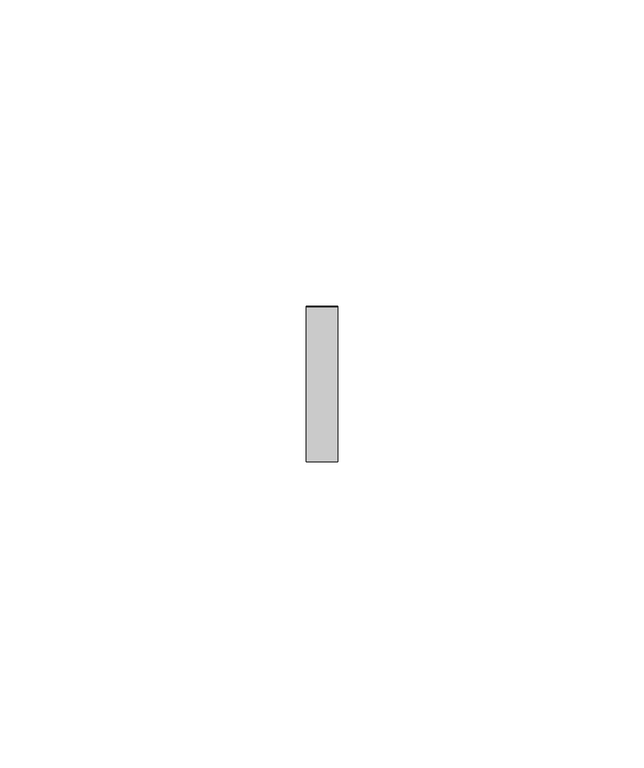
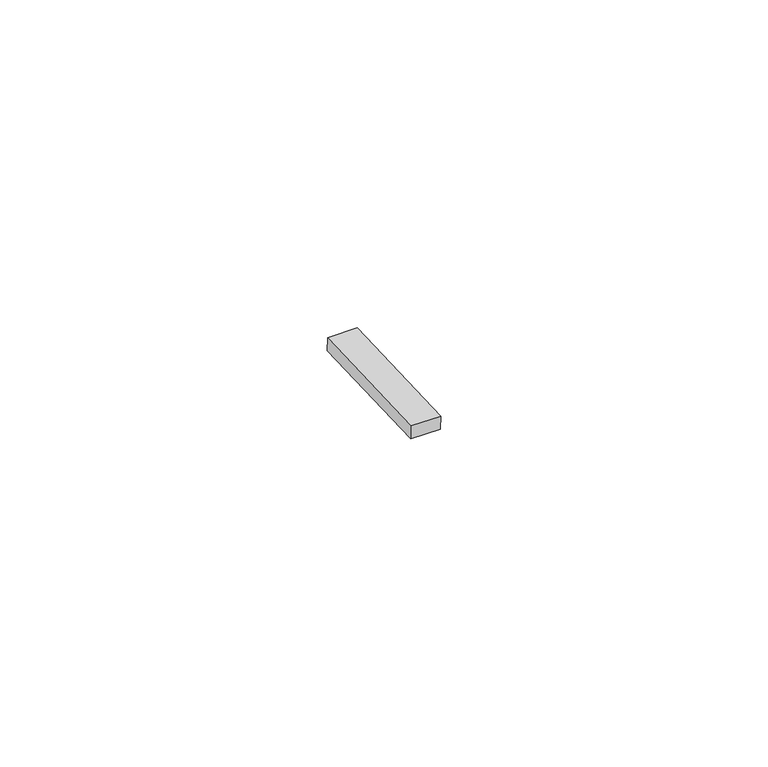
"""IFC4 building model written with IfcOpenShell, lengths in millimetres: proxy geometry, Inner panel:Inner panel:1:Inner panel:1 : Inner panel:Inner panel:300324:2:Inner panel:1:Inner panel:1 : Inner panel:Inner panel:300324:2 : Inner panel:Inner panel:1:Inner panel:1 : Inner panel:Inner panel:300324:300043:137 : Inner panel:Inner panel:1:Inner panel:1 : Inner panel:Inner panel:300324:2:Inner panel:1:Inner panel:1 : Inner panel:Inner panel:300324:2 : Inner panel:Inner panel:1:Inner panel:1 : Inner panel:Inner panel:300324:300043:308120."""

import ifcopenshell
import ifcopenshell.guid

model = None  # the IFC model being written
_history = None  # IfcOwnerHistory: only IFC2X3 demands one
_inside = {}  # id of a spatial element -> (the spatial element, [elements in it])
_under = {}  # id of a project, library or spatial element -> (it, [spatial elements below it])
_declared = {}  # id of a project -> (the project, [libraries it declares])
_typed = {}  # id of a type object -> (the type object, [elements of that type])
_made_of = {}  # id of a material, layer set ... -> (it, [elements and type objects made of it])


def new_model(schema):
    """Start an empty IFC model of exactly this schema.

    Asked for "IFC4X3", IfcOpenShell would pick the latest addendum, in which some entities
    have other attributes; the version numbers below select the first issue.
    IFC2X3 requires an IfcOwnerHistory on every rooted entity: one is made here for all.
    """
    global model, _history
    if schema == "IFC4X3":
        model = ifcopenshell.file(schema_version=(4, 3, 0, 0))
    else:
        model = ifcopenshell.file(schema=schema)
    _inside.clear()
    _under.clear()
    _declared.clear()
    _typed.clear()
    _made_of.clear()
    _history = None
    if model.schema == "IFC2X3":
        org = make("IfcOrganization", Name="unknown")
        user = make(
            "IfcPersonAndOrganization",
            ThePerson=make("IfcPerson", FamilyName="unknown"),
            TheOrganization=org,
        )
        app = make(
            "IfcApplication",
            ApplicationDeveloper=org,
            Version="unknown",
            ApplicationFullName="unknown",
            ApplicationIdentifier="unknown",
        )
        _history = make(
            "IfcOwnerHistory",
            OwningUser=user,
            OwningApplication=app,
            ChangeAction="ADDED",
            CreationDate=0,
        )
    return model


def make(cls, **values):
    """One entity of the class cls with the attributes given. An attribute that is None is left unset."""
    return model.create_entity(
        cls, **{name: value for name, value in values.items() if value is not None}
    )


def rooted(cls, **values):
    """An entity with a GlobalId (a new one), such as an element, a storey or a relation."""
    return make(cls, GlobalId=ifcopenshell.guid.new(), OwnerHistory=_history, **values)


def si_unit(unit_type, name, prefix=None):
    """IfcSIUnit, for example si_unit("LENGTHUNIT", "METRE", prefix="MILLI")."""
    return make("IfcSIUnit", UnitType=unit_type, Prefix=prefix, Name=name)


def assignment(units):
    """IfcUnitAssignment: the units of a project."""
    return None if units is None else make("IfcUnitAssignment", Units=units)


def point(xyz):
    """IfcCartesianPoint."""
    return None if xyz is None else make("IfcCartesianPoint", Coordinates=xyz)


def direction(xyz):
    """IfcDirection."""
    return None if xyz is None else make("IfcDirection", DirectionRatios=xyz)


def frame(location, z_axis=None, x_axis=None):
    """IfcAxis2Placement3D, a coordinate frame: its origin and axes. An axis left out is left unset."""
    return make(
        "IfcAxis2Placement3D",
        Location=point(location),
        Axis=direction(z_axis),
        RefDirection=direction(x_axis),
    )


def origin():
    """The frame at (0, 0, 0) with its axes left unset."""
    return frame((0.0, 0.0, 0.0))


def place(relative_to, where):
    """IfcLocalPlacement: puts the frame where relative to a parent placement (None: the world)."""
    return make(
        "IfcLocalPlacement", PlacementRelTo=relative_to, RelativePlacement=where
    )


def context(
    kind, dimensions, precision=None, world=None, true_north=None, identifier=None
):
    """IfcGeometricRepresentationContext, for example the 3D "Model" context."""
    return make(
        "IfcGeometricRepresentationContext",
        ContextIdentifier=identifier,
        ContextType=kind,
        CoordinateSpaceDimension=dimensions,
        Precision=precision,
        WorldCoordinateSystem=world,
        TrueNorth=true_north,
    )


def project(units=None, contexts=None):
    """IfcProject with its units and contexts."""
    return rooted(
        "IfcProject",
        Name="project",
        RepresentationContexts=contexts,
        UnitsInContext=assignment(units),
    )


def spatial(cls, under=None, at=None, **own):
    """A site, building, storey or space (cls), placed at a placement, below another one or the project."""
    s = rooted(cls, ObjectPlacement=at, **own)
    if under is not None:
        _under.setdefault(under.id(), (under, []))[1].append(s)
    return s


def polyline(points):
    """IfcPolyline through the points."""
    return make("IfcPolyline", Points=[point(p) for p in points])


def outline(outer, holes=None, kind="AREA"):
    """IfcArbitraryClosedProfileDef: a profile drawn as a closed curve; with holes, ...WithVoids."""
    if holes is None:
        return make("IfcArbitraryClosedProfileDef", ProfileType=kind, OuterCurve=outer)
    return make(
        "IfcArbitraryProfileDefWithVoids",
        ProfileType=kind,
        OuterCurve=outer,
        InnerCurves=holes,
    )


def extrude(swept, where, along, depth):
    """IfcExtrudedAreaSolid: the profile swept, set in the frame where, extruded along a direction by depth."""
    return make(
        "IfcExtrudedAreaSolid",
        SweptArea=swept,
        Position=where,
        ExtrudedDirection=direction(along),
        Depth=depth,
    )


def shape(context_of_items, identifier, shape_type, items):
    """IfcShapeRepresentation: the items that make up one representation, for example the "Body"."""
    return make(
        "IfcShapeRepresentation",
        ContextOfItems=context_of_items,
        RepresentationIdentifier=identifier,
        RepresentationType=shape_type,
        Items=items,
    )


def source(mapping_origin, context_of_items, identifier, shape_type, items):
    """IfcRepresentationMap: a shape defined once, which mapped items show again and again."""
    return make(
        "IfcRepresentationMap",
        MappingOrigin=mapping_origin,
        MappedRepresentation=shape(context_of_items, identifier, shape_type, items),
    )


def transform(
    local_origin,
    x_axis=None,
    y_axis=None,
    z_axis=None,
    scale=None,
    scale2=None,
    scale3=None,
    uniform=True,
):
    """IfcCartesianTransformationOperator3D, or its non-uniform kind. x_axis, y_axis, z_axis: its Axis1, 2, 3."""
    if uniform:
        return make(
            "IfcCartesianTransformationOperator3D",
            Axis1=direction(x_axis),
            Axis2=direction(y_axis),
            LocalOrigin=point(local_origin),
            Scale=scale,
            Axis3=direction(z_axis),
        )
    return make(
        "IfcCartesianTransformationOperator3DnonUniform",
        Axis1=direction(x_axis),
        Axis2=direction(y_axis),
        LocalOrigin=point(local_origin),
        Scale=scale,
        Axis3=direction(z_axis),
        Scale2=scale2,
        Scale3=scale3,
    )


def mapped(mapping_source, mapping_target):
    """IfcMappedItem: shows the shape of a source again, moved by a transform."""
    return make(
        "IfcMappedItem", MappingSource=mapping_source, MappingTarget=mapping_target
    )


def made_of(thing, what):
    """Note that an element or type object is made of a material, layer set ...; save() writes the relation."""
    if what is not None:
        _made_of.setdefault(what.id(), (what, []))[1].append(thing)
    return thing


def element(
    cls,
    number,
    at=None,
    inside=None,
    cuts=None,
    type_object=None,
    material=None,
    context=None,
    identifier="Body",
    shape_type=None,
    held_by="IfcProductDefinitionShape",
    body=None,
    shapes=None,
    **own,
):
    """One element of the class cls, such as IfcWall. Its Tag is "e" and its number.

    at: its placement. inside: the storey or other place that contains it. cuts: it is an
    opening in that element (IfcRelVoidsElement). A single representation is given by context,
    identifier, shape_type and body (its items); several are given by shapes. held_by: the class
    of the entity that holds the representations. save() writes the other relations.
    """
    e = rooted(cls, Tag="e%d" % number, ObjectPlacement=at, **own)
    if body is not None:
        shapes = [shape(context, identifier, shape_type, body)]
    if shapes is not None:
        e.Representation = make(held_by, Representations=shapes)
    if inside is not None:
        _inside.setdefault(inside.id(), (inside, []))[1].append(e)
    if cuts is not None:
        rooted(
            "IfcRelVoidsElement", RelatingBuildingElement=cuts, RelatedOpeningElement=e
        )
    if type_object is not None:
        _typed.setdefault(type_object.id(), (type_object, []))[1].append(e)
    return made_of(e, material)


def aggregate(whole, parts):
    """IfcRelAggregates: a whole, such as a stair, and the parts it consists of."""
    return rooted("IfcRelAggregates", RelatingObject=whole, RelatedObjects=parts)


def save(model, path):
    """Write the relations noted so far, then the file.

    IfcRelAggregates (storeys below a building ...), IfcRelContainedInSpatialStructure (elements
    in a storey), IfcRelDefinesByType, IfcRelAssociatesMaterial and IfcRelDeclares: one each for
    every whole, place, type object, material and project.
    """
    for whole, parts in _under.values():
        aggregate(whole, parts)
    for where, things in _inside.values():
        rooted(
            "IfcRelContainedInSpatialStructure",
            RelatedElements=things,
            RelatingStructure=where,
        )
    for kind, things in _typed.values():
        rooted("IfcRelDefinesByType", RelatedObjects=things, RelatingType=kind)
    for what, things in _made_of.values():
        rooted("IfcRelAssociatesMaterial", RelatedObjects=things, RelatingMaterial=what)
    for by, libraries in _declared.values():
        rooted("IfcRelDeclares", RelatingContext=by, RelatedDefinitions=libraries)
    model.write(path)


def generic_models_5d017d1f(model_context):
    return source(origin(), model_context, "Body", "SweptSolid", [
        extrude(outline(polyline([(0.0, -25.3999999), (0.0, 0.0), (5.2138089, 0.0), (5.2138089, -25.3999999), (0.0, -25.3999999)])), frame((591904.595117, -568123.7593241, 8806.3160403), z_axis=(0.0, -0.041630544712223896, 0.9991330730923502), x_axis=(-1.0, 0.0, 0.0)), (0.0, 0.0, 1.0), 2.4763745),
    ])


if __name__ == "__main__":
    model = new_model("IFC4")
    model_context = context("Model", 3, world=origin())
    ifc_project = project(units=[si_unit("LENGTHUNIT", "METRE", prefix="MILLI")], contexts=[model_context])
    site = spatial("IfcSite", under=ifc_project)
    building = spatial("IfcBuilding", under=site)
    placement = place(None, origin())
    generic_models_shape = generic_models_5d017d1f(model_context)
    element("IfcBuildingElementProxy", 1, Name="Inner panel:Inner panel:1:Inner panel:1 : Inner panel:Inner panel:300324:2:Inner panel:1:Inner panel:1 : Inner panel:Inner panel:300324:2 : Inner panel:Inner panel:1:Inner panel:1 : Inner panel:Inner panel:300324:300043:137 : Inner panel:Inner panel:1:Inner panel:1 : Inner panel:Inner panel:300324:2:Inner panel:1:Inner panel:1 : Inner panel:Inner panel:300324:2 : Inner panel:Inner panel:1:Inner panel:1 : Inner panel:Inner panel:300324:300043:308120", ObjectType="Inner panel:Inner panel:1:Inner panel:1 : Inner panel:Inner panel:300324:2:Inner panel:1:Inner panel:1 : Inner panel:Inner panel:300324:2 : Inner panel:Inner panel:1:Inner panel:1 : Inner panel:Inner panel:300324:300043:137 : Inner panel:Inner panel:1:Inner panel:1 : Inner panel:Inner panel:300324:2:Inner panel:1:Inner panel:1 : Inner panel:Inner panel:300324:2 : Inner panel:Inner panel:1:Inner panel:1 : Inner panel:Inner panel:300324:300043:308120", at=placement, inside=building, context=model_context, shape_type="MappedRepresentation", body=[
        mapped(generic_models_shape, transform((0.0, 0.0, 0.0), x_axis=(1.0, 0.0, 0.0), y_axis=(0.0, 1.0, 0.0), z_axis=(0.0, 0.0, 1.0))),
    ])
    save(model, "model.ifc")

# Revit data of these elements
# Type "Inner panel:Inner panel:1:Inner panel:1 : Inner panel:Inner panel:300324:2:Inner panel:1:Inner panel:1 : Inner panel:Inner panel:300324:2 : Inner panel:Inner panel:1:Inner panel:1 : Inner panel:Inner panel:300324:300043:137 : Inner panel:Inner panel:1:Inner panel:1 : Inner panel:Inner panel:300324:2:Inner panel:1:Inner panel:1 : Inner panel:Inner panel:300324:2 : Inner panel:Inner panel:1:Inner panel:1 : Inner panel:Inner panel:300324:300043:308120"
#   NameOverride = "Inner panel:Inner panel:1:Inner panel:1 : Inner panel:Inner panel:300324:2:Inner panel:1:Inner panel:1 : Inner panel:Inner panel:300324:2 : Inner panel:Inner panel:1:Inner panel:1 : Inner panel:Inner panel:300324:300043:308120"
#   ObjectTypeOverride = "Inner panel:1:Inner panel:1 : Inner panel:Inner panel:300324:2 : Inner panel:Inner panel:1:Inner panel:1 : Inner panel:Inner panel:300324:300043"
#   Reference = "Inner panel"
#   Tag = "308120"
# Element 1 (IfcBuildingElementProxy, "Inner panel:Inner panel:1:Inner panel:1 : Inner panel:Inner panel:300324:2:Inner panel:1:Inner panel:1 : Inner panel:Inner panel:300324:2 : Inner panel:Inner panel:1:Inner panel:1 : Inner panel:Inner panel:300324:300043:137 : Inner panel:Inner panel:1:Inner panel:1 : Inner panel:Inner panel:300324:2:Inner panel:1:Inner panel:1 : Inner panel:Inner panel:300324:2 : Inner panel:Inner panel:1:Inner panel:1 : Inner panel:Inner panel:300324:300043:308120")
#   Materials on its faces: "AT CLIP - 1\" WIDE NON ABSORBENT, WEATHER-RESISTANT NEOPRENE/EPDM/SBR FOAM"
# Materials
#   "AT CLIP - 1\" WIDE NON ABSORBENT, WEATHER-RESISTANT NEOPRENE/EPDM/SBR FOAM": class "Generic", colour RGB 85 85 85, transparency 0, Cost = 0
